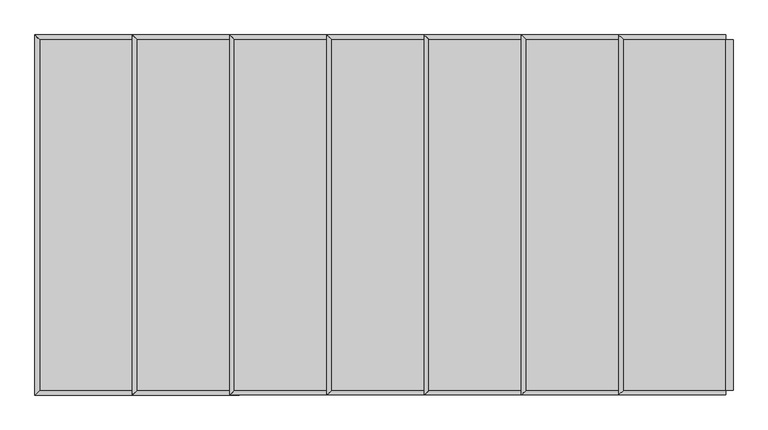
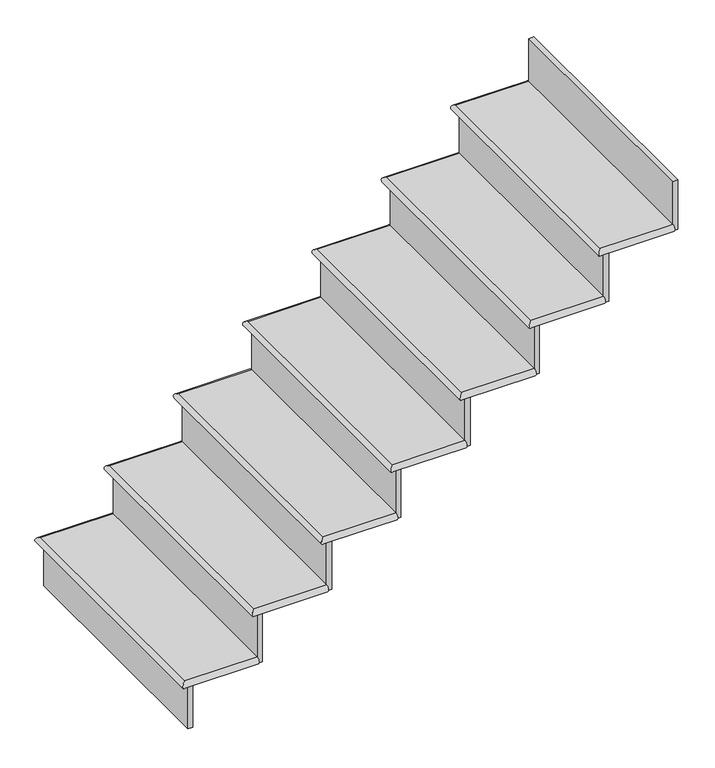
"""IFC4 building model written with IfcOpenShell, lengths in millimetres: stair flight geometry."""

import ifcopenshell
import ifcopenshell.guid

model = None  # the IFC model being written
_history = None  # IfcOwnerHistory: only IFC2X3 demands one
_inside = {}  # id of a spatial element -> (the spatial element, [elements in it])
_under = {}  # id of a project, library or spatial element -> (it, [spatial elements below it])
_declared = {}  # id of a project -> (the project, [libraries it declares])
_typed = {}  # id of a type object -> (the type object, [elements of that type])
_made_of = {}  # id of a material, layer set ... -> (it, [elements and type objects made of it])


def new_model(schema):
    """Start an empty IFC model of exactly this schema.

    Asked for "IFC4X3", IfcOpenShell would pick the latest addendum, in which some entities
    have other attributes; the version numbers below select the first issue.
    IFC2X3 requires an IfcOwnerHistory on every rooted entity: one is made here for all.
    """
    global model, _history
    if schema == "IFC4X3":
        model = ifcopenshell.file(schema_version=(4, 3, 0, 0))
    else:
        model = ifcopenshell.file(schema=schema)
    _inside.clear()
    _under.clear()
    _declared.clear()
    _typed.clear()
    _made_of.clear()
    _history = None
    if model.schema == "IFC2X3":
        org = make("IfcOrganization", Name="unknown")
        user = make(
            "IfcPersonAndOrganization",
            ThePerson=make("IfcPerson", FamilyName="unknown"),
            TheOrganization=org,
        )
        app = make(
            "IfcApplication",
            ApplicationDeveloper=org,
            Version="unknown",
            ApplicationFullName="unknown",
            ApplicationIdentifier="unknown",
        )
        _history = make(
            "IfcOwnerHistory",
            OwningUser=user,
            OwningApplication=app,
            ChangeAction="ADDED",
            CreationDate=0,
        )
    return model


def make(cls, **values):
    """One entity of the class cls with the attributes given. An attribute that is None is left unset."""
    return model.create_entity(
        cls, **{name: value for name, value in values.items() if value is not None}
    )


def rooted(cls, **values):
    """An entity with a GlobalId (a new one), such as an element, a storey or a relation."""
    return make(cls, GlobalId=ifcopenshell.guid.new(), OwnerHistory=_history, **values)


def si_unit(unit_type, name, prefix=None):
    """IfcSIUnit, for example si_unit("LENGTHUNIT", "METRE", prefix="MILLI")."""
    return make("IfcSIUnit", UnitType=unit_type, Prefix=prefix, Name=name)


def assignment(units):
    """IfcUnitAssignment: the units of a project."""
    return None if units is None else make("IfcUnitAssignment", Units=units)


def point(xyz):
    """IfcCartesianPoint."""
    return None if xyz is None else make("IfcCartesianPoint", Coordinates=xyz)


def direction(xyz):
    """IfcDirection."""
    return None if xyz is None else make("IfcDirection", DirectionRatios=xyz)


def frame(location, z_axis=None, x_axis=None):
    """IfcAxis2Placement3D, a coordinate frame: its origin and axes. An axis left out is left unset."""
    return make(
        "IfcAxis2Placement3D",
        Location=point(location),
        Axis=direction(z_axis),
        RefDirection=direction(x_axis),
    )


def origin():
    """The frame at (0, 0, 0) with its axes left unset."""
    return frame((0.0, 0.0, 0.0))


def place(relative_to, where):
    """IfcLocalPlacement: puts the frame where relative to a parent placement (None: the world)."""
    return make(
        "IfcLocalPlacement", PlacementRelTo=relative_to, RelativePlacement=where
    )


def context(
    kind, dimensions, precision=None, world=None, true_north=None, identifier=None
):
    """IfcGeometricRepresentationContext, for example the 3D "Model" context."""
    return make(
        "IfcGeometricRepresentationContext",
        ContextIdentifier=identifier,
        ContextType=kind,
        CoordinateSpaceDimension=dimensions,
        Precision=precision,
        WorldCoordinateSystem=world,
        TrueNorth=true_north,
    )


def project(units=None, contexts=None):
    """IfcProject with its units and contexts."""
    return rooted(
        "IfcProject",
        Name="project",
        RepresentationContexts=contexts,
        UnitsInContext=assignment(units),
    )


def spatial(cls, under=None, at=None, **own):
    """A site, building, storey or space (cls), placed at a placement, below another one or the project."""
    s = rooted(cls, ObjectPlacement=at, **own)
    if under is not None:
        _under.setdefault(under.id(), (under, []))[1].append(s)
    return s


def circle_curve(where, radius):
    """IfcCircle in the frame where."""
    return make("IfcCircle", Position=where, Radius=radius)


def ellipse_curve(where, semi_axis1, semi_axis2):
    """IfcEllipse in the frame where."""
    return make(
        "IfcEllipse", Position=where, SemiAxis1=semi_axis1, SemiAxis2=semi_axis2
    )


def faces_of(points, faces, orient=None, outer=None):
    """IfcFace entities. A face is a list of loops; a loop is a list of indices into points, from 0.

    orient and outer hold one flag for each loop. By default every Orientation is true, the
    first loop of a face is its IfcFaceOuterBound and the others are IfcFaceBound.
    """
    made = []
    for i, loops in enumerate(faces):
        bounds = []
        for j, loop in enumerate(loops):
            is_outer = j == 0 if outer is None else outer[i][j]
            bounds.append(
                make(
                    "IfcFaceOuterBound" if is_outer else "IfcFaceBound",
                    Bound=make("IfcPolyLoop", Polygon=[points[k] for k in loop]),
                    Orientation=True if orient is None else orient[i][j],
                )
            )
        made.append(make("IfcFace", Bounds=bounds))
    return made


def faceted_brep(points, faces, orient=None, outer=None, voids=None):
    """IfcFacetedBrep: a solid bounded by flat faces; with voids (closed shells), ...WithVoids."""
    shared = [point(p) for p in points]
    hull = make("IfcClosedShell", CfsFaces=faces_of(shared, faces, orient, outer))
    if voids is None:
        return make("IfcFacetedBrep", Outer=hull)
    return make(
        "IfcFacetedBrepWithVoids",
        Outer=hull,
        Voids=[
            make(cls, CfsFaces=faces_of(shared, fs, o, b)) for cls, fs, o, b in voids
        ],
    )


def shape(context_of_items, identifier, shape_type, items):
    """IfcShapeRepresentation: the items that make up one representation, for example the "Body"."""
    return make(
        "IfcShapeRepresentation",
        ContextOfItems=context_of_items,
        RepresentationIdentifier=identifier,
        RepresentationType=shape_type,
        Items=items,
    )


def source(mapping_origin, context_of_items, identifier, shape_type, items):
    """IfcRepresentationMap: a shape defined once, which mapped items show again and again."""
    return make(
        "IfcRepresentationMap",
        MappingOrigin=mapping_origin,
        MappedRepresentation=shape(context_of_items, identifier, shape_type, items),
    )


def transform(
    local_origin,
    x_axis=None,
    y_axis=None,
    z_axis=None,
    scale=None,
    scale2=None,
    scale3=None,
    uniform=True,
):
    """IfcCartesianTransformationOperator3D, or its non-uniform kind. x_axis, y_axis, z_axis: its Axis1, 2, 3."""
    if uniform:
        return make(
            "IfcCartesianTransformationOperator3D",
            Axis1=direction(x_axis),
            Axis2=direction(y_axis),
            LocalOrigin=point(local_origin),
            Scale=scale,
            Axis3=direction(z_axis),
        )
    return make(
        "IfcCartesianTransformationOperator3DnonUniform",
        Axis1=direction(x_axis),
        Axis2=direction(y_axis),
        LocalOrigin=point(local_origin),
        Scale=scale,
        Axis3=direction(z_axis),
        Scale2=scale2,
        Scale3=scale3,
    )


def mapped(mapping_source, mapping_target):
    """IfcMappedItem: shows the shape of a source again, moved by a transform."""
    return make(
        "IfcMappedItem", MappingSource=mapping_source, MappingTarget=mapping_target
    )


def made_of(thing, what):
    """Note that an element or type object is made of a material, layer set ...; save() writes the relation."""
    if what is not None:
        _made_of.setdefault(what.id(), (what, []))[1].append(thing)
    return thing


def element(
    cls,
    number,
    at=None,
    inside=None,
    cuts=None,
    type_object=None,
    material=None,
    context=None,
    identifier="Body",
    shape_type=None,
    held_by="IfcProductDefinitionShape",
    body=None,
    shapes=None,
    **own,
):
    """One element of the class cls, such as IfcWall. Its Tag is "e" and its number.

    at: its placement. inside: the storey or other place that contains it. cuts: it is an
    opening in that element (IfcRelVoidsElement). A single representation is given by context,
    identifier, shape_type and body (its items); several are given by shapes. held_by: the class
    of the entity that holds the representations. save() writes the other relations.
    """
    e = rooted(cls, Tag="e%d" % number, ObjectPlacement=at, **own)
    if body is not None:
        shapes = [shape(context, identifier, shape_type, body)]
    if shapes is not None:
        e.Representation = make(held_by, Representations=shapes)
    if inside is not None:
        _inside.setdefault(inside.id(), (inside, []))[1].append(e)
    if cuts is not None:
        rooted(
            "IfcRelVoidsElement", RelatingBuildingElement=cuts, RelatedOpeningElement=e
        )
    if type_object is not None:
        _typed.setdefault(type_object.id(), (type_object, []))[1].append(e)
    return made_of(e, material)


def aggregate(whole, parts):
    """IfcRelAggregates: a whole, such as a stair, and the parts it consists of."""
    return rooted("IfcRelAggregates", RelatingObject=whole, RelatedObjects=parts)


def save(model, path):
    """Write the relations noted so far, then the file.

    IfcRelAggregates (storeys below a building ...), IfcRelContainedInSpatialStructure (elements
    in a storey), IfcRelDefinesByType, IfcRelAssociatesMaterial and IfcRelDeclares: one each for
    every whole, place, type object, material and project.
    """
    for whole, parts in _under.values():
        aggregate(whole, parts)
    for where, things in _inside.values():
        rooted(
            "IfcRelContainedInSpatialStructure",
            RelatedElements=things,
            RelatingStructure=where,
        )
    for kind, things in _typed.values():
        rooted("IfcRelDefinesByType", RelatedObjects=things, RelatingType=kind)
    for what, things in _made_of.values():
        rooted("IfcRelAssociatesMaterial", RelatedObjects=things, RelatingMaterial=what)
    for by, libraries in _declared.values():
        rooted("IfcRelDeclares", RelatingContext=by, RelatedDefinitions=libraries)
    model.write(path)


def plane_surface(at):
    """IfcPlane: the flat surface through the origin of the frame at, square to its z axis."""
    return make("IfcPlane", Position=at)


def cylinder_surface(at, radius):
    """IfcCylindricalSurface: all points at the distance radius from the z axis of the frame at."""
    return make("IfcCylindricalSurface", Position=at, Radius=radius)


def advanced_brep(points, edges, surfaces, faces):
    """IfcAdvancedBrep: a solid bounded by faces that lie on surfaces and meet in shared edges.

    An edge is (start, end): straight between two places in points (the first is 0);
    or (start, end, curve); or (start, end, curve, False) where it runs against its curve.
    A face is (place in surfaces, loops), or (place, loops, False) where it looks against
    its surface's normal. A loop lists edges by number (the first is 1), with a minus sign
    where the edge is run from its end to its start. The first loop is the outer one.
    """
    corners = [point(p) for p in points]
    vertices = [make("IfcVertexPoint", VertexGeometry=c) for c in corners]
    made = []
    for start, end, *more in edges:
        made.append(
            make(
                "IfcEdgeCurve",
                EdgeStart=vertices[start],
                EdgeEnd=vertices[end],
                EdgeGeometry=more[0] if more else make("IfcPolyline", Points=[corners[start], corners[end]]),
                SameSense=more[1] if len(more) > 1 else True,
            )
        )
    hull = []
    for where, loops, *sense in faces:
        bounds = []
        for j, loop in enumerate(loops):
            ring = [make("IfcOrientedEdge", EdgeElement=made[abs(k) - 1], Orientation=k > 0) for k in loop]
            bounds.append(
                make(
                    "IfcFaceOuterBound" if j == 0 else "IfcFaceBound",
                    Bound=make("IfcEdgeLoop", EdgeList=ring),
                    Orientation=True,
                )
            )
        hull.append(make("IfcAdvancedFace", Bounds=bounds, FaceSurface=surfaces[where], SameSense=sense[0] if sense else True))
    return make("IfcAdvancedBrep", Outer=make("IfcClosedShell", CfsFaces=hull))


def stair_flight_e1e404fc(model_context):
    return source(origin(), model_context, "Body", "SolidModel", [
        advanced_brep(
        [(-17769.3481446, 3955.9128094, 165.1), (-17769.3481446, 3955.9128094, 190.5), (-17769.3481446, 4870.3128094, 190.5), (-17769.3481446, 4870.3128094, 165.1), (-17502.6481446, 3955.9128094, 190.5), (-17502.6481446, 4870.3128094, 190.5), (-17502.6481446, 4870.3128094, 165.1), (-17502.6481446, 3955.9128094, 165.1)],
        [
            (0, 1, ellipse_curve(frame((-17769.3481446, 3955.9128094, 177.8), z_axis=(-0.7071067811865449, 0.7071067811865502, 0.0), x_axis=(-0.7071067811865503, -0.7071067811865447, 0.0)), 17.9605122, 12.7)),
            (1, 2),
            (2, 3, ellipse_curve(frame((-17769.3481446, 4870.3128094, 177.8), z_axis=(-0.7071067811865501, -0.7071067811865447, 0.0), x_axis=(0.7071067811865446, -0.7071067811865506, 0.0)), 17.9605122, 12.7)),
            (3, 0),
            (4, 5),
            (5, 2),
            (1, 4),
            (6, 7),
            (7, 0),
            (3, 6),
            (4, 7, circle_curve(frame((-17502.6481446, 3955.9128094, 177.8), z_axis=(1.0, 0.0, 0.0), x_axis=(0.0, 1.0, 0.0)), 12.7)),
            (6, 5, circle_curve(frame((-17502.6481446, 4870.3128094, 177.8), z_axis=(1.0, 0.0, 0.0), x_axis=(0.0, -1.0, 0.0)), 12.7)),
        ],
        [
            cylinder_surface(frame((-17769.3481446, 3955.9128094, 177.8), z_axis=(0.0, -1.0, 0.0), x_axis=(1.0, 0.0, 0.0)), 12.7),
            plane_surface(frame((-17782.0481446, 4870.3128094, 190.5), z_axis=(0.0, 0.0, 1.0), x_axis=(-1.0, 0.0, 0.0))),
            plane_surface(frame((-17782.0481446, 4870.3128094, 165.1), z_axis=(0.0, 0.0, -1.0), x_axis=(1.0, 0.0, 0.0))),
            plane_surface(frame((-17502.6481446, 3955.9128094, 190.5), z_axis=(1.0, 0.0, 0.0), x_axis=(0.0, 0.0, -1.0))),
            cylinder_surface(frame((-17502.6481446, 3955.9128094, 177.8), z_axis=(1.0, 0.0, 0.0), x_axis=(0.0, 1.0, 0.0)), 12.7),
            cylinder_surface(frame((-17769.3481446, 4870.3128094, 177.8), z_axis=(-1.0, 0.0, 0.0), x_axis=(0.0, -1.0, 0.0)), 12.7),
        ],
        [
            (0, [[1, 2, 3, 4]]),
            (1, [[5, 6, -2, 7]]),
            (2, [[8, 9, -4, 10]]),
            (3, [[-5, 11, -8, 12]]),
            (4, [[-11, -7, -1, -9]]),
            (5, [[-3, -6, -12, -10]]),
        ],
    ),
        faceted_brep([(-17756.6481446, 3955.9128094, 165.1), (-17756.6481446, 3955.9128094, 0.0), (-17737.5981446, 3955.9128094, 0.0), (-17737.5981446, 3955.9128094, 165.1), (-17756.6481446, 4870.3128094, 165.1), (-17737.5981446, 4870.3128094, 165.1), (-17737.5981446, 4870.3128094, 0.0), (-17756.6481446, 4870.3128094, 0.0)], [[[0, 1, 2, 3]], [[4, 5, 6, 7]], [[1, 0, 4, 7]], [[2, 1, 7, 6]], [[3, 2, 6, 5]], [[0, 3, 5, 4]]]),
        faceted_brep([(-17502.6481446, 3955.9128094, 355.6), (-17502.6481446, 3955.9128094, 165.1), (-17483.5981446, 3955.9128094, 165.1), (-17483.5981446, 3955.9128094, 355.6), (-17502.6481446, 4870.3128094, 355.6), (-17483.5981446, 4870.3128094, 355.6), (-17483.5981446, 4870.3128094, 165.1), (-17502.6481446, 4870.3128094, 165.1)], [[[0, 1, 2, 3]], [[4, 5, 6, 7]], [[1, 0, 4, 7]], [[2, 1, 7, 6]], [[3, 2, 6, 5]], [[0, 3, 5, 4]]]),
        advanced_brep(
        [(-17248.6481446, 3955.9128094, 381.0), (-17248.6481446, 4870.3128094, 381.0), (-17515.3481446, 4870.3128094, 381.0), (-17515.3481446, 3955.9128094, 381.0), (-17248.6481446, 4870.3128094, 355.6), (-17248.6481446, 3955.9128094, 355.6), (-17515.3481446, 3955.9128094, 355.6), (-17515.3481446, 4870.3128094, 355.6)],
        [
            (0, 1),
            (1, 2),
            (2, 3),
            (3, 0),
            (4, 5),
            (5, 6),
            (6, 7),
            (7, 4),
            (0, 5, circle_curve(frame((-17248.6481446, 3955.9128094, 368.3), z_axis=(1.0, 0.0, 0.0), x_axis=(0.0, 1.0, 0.0)), 12.7)),
            (4, 1, circle_curve(frame((-17248.6481446, 4870.3128094, 368.3), z_axis=(1.0, 0.0, 0.0), x_axis=(0.0, -1.0, 0.0)), 12.7)),
            (6, 3, ellipse_curve(frame((-17515.3481446, 3955.9128094, 368.3), z_axis=(-0.7071067811865457, 0.7071067811865495, 0.0), x_axis=(-0.7071067811865496, -0.7071067811865455, 0.0)), 17.9605122, 12.7)),
            (2, 7, ellipse_curve(frame((-17515.3481446, 4870.3128094, 368.3), z_axis=(-0.7071067811865496, -0.7071067811865455, 0.0), x_axis=(0.7071067811865455, -0.7071067811865496, 0.0)), 17.9605122, 12.7)),
        ],
        [
            plane_surface(frame((-17782.0481446, 4870.3128094, 381.0), z_axis=(0.0, 0.0, 1.0), x_axis=(-1.0, 0.0, 0.0))),
            plane_surface(frame((-17782.0481446, 4870.3128094, 355.6), z_axis=(0.0, 0.0, -1.0), x_axis=(1.0, 0.0, 0.0))),
            plane_surface(frame((-17248.6481446, 3955.9128094, 381.0), z_axis=(1.0, 0.0, 0.0), x_axis=(0.0, 0.0, -1.0))),
            cylinder_surface(frame((-17515.3481446, 3955.9128094, 368.3), z_axis=(0.0, -1.0, 0.0), x_axis=(1.0, 0.0, 0.0)), 12.7),
            cylinder_surface(frame((-17248.6481446, 3955.9128094, 368.3), z_axis=(1.0, 0.0, 0.0), x_axis=(0.0, 1.0, 0.0)), 12.7),
            cylinder_surface(frame((-17515.3481446, 4870.3128094, 368.3), z_axis=(-1.0, 0.0, 0.0), x_axis=(0.0, -1.0, 0.0)), 12.7),
        ],
        [
            (0, [[1, 2, 3, 4]]),
            (1, [[5, 6, 7, 8]]),
            (2, [[-1, 9, -5, 10]]),
            (3, [[11, -3, 12, -7]]),
            (4, [[-9, -4, -11, -6]]),
            (5, [[-12, -2, -10, -8]]),
        ],
    ),
        faceted_brep([(-17248.6481446, 3955.9128094, 546.1), (-17248.6481446, 3955.9128094, 355.6), (-17229.5981446, 3955.9128094, 355.6), (-17229.5981446, 3955.9128094, 546.1), (-17248.6481446, 4870.3128094, 546.1), (-17229.5981446, 4870.3128094, 546.1), (-17229.5981446, 4870.3128094, 355.6), (-17248.6481446, 4870.3128094, 355.6)], [[[0, 1, 2, 3]], [[4, 5, 6, 7]], [[1, 0, 4, 7]], [[2, 1, 7, 6]], [[3, 2, 6, 5]], [[0, 3, 5, 4]]]),
        advanced_brep(
        [(-16994.6481446, 3955.9128094, 571.5), (-16994.6481446, 4870.3128094, 571.5), (-17261.3481446, 4870.3128094, 571.5), (-17261.3481446, 3955.9128094, 571.5), (-16994.6481446, 4870.3128094, 546.1), (-16994.6481446, 3955.9128094, 546.1), (-17261.3481446, 3955.9128094, 546.1), (-17261.3481446, 4870.3128094, 546.1)],
        [
            (0, 1),
            (1, 2),
            (2, 3),
            (3, 0),
            (4, 5),
            (5, 6),
            (6, 7),
            (7, 4),
            (0, 5, circle_curve(frame((-16994.6481446, 3955.9128094, 558.8), z_axis=(1.0, 0.0, 0.0), x_axis=(0.0, 1.0, 0.0)), 12.7)),
            (4, 1, circle_curve(frame((-16994.6481446, 4870.3128094, 558.8), z_axis=(1.0, 0.0, 0.0), x_axis=(0.0, -1.0, 0.0)), 12.7)),
            (6, 3, ellipse_curve(frame((-17261.3481446, 3955.9128094, 558.8), z_axis=(-0.7071067811865457, 0.7071067811865495, 0.0), x_axis=(-0.7071067811865496, -0.7071067811865455, 0.0)), 17.9605122, 12.7)),
            (2, 7, ellipse_curve(frame((-17261.3481446, 4870.3128094, 558.8), z_axis=(-0.7071067811865496, -0.7071067811865455, 0.0), x_axis=(0.7071067811865455, -0.7071067811865496, 0.0)), 17.9605122, 12.7)),
        ],
        [
            plane_surface(frame((-17528.0481446, 4870.3128094, 571.5), z_axis=(0.0, 0.0, 1.0), x_axis=(-1.0, 0.0, 0.0))),
            plane_surface(frame((-17528.0481446, 4870.3128094, 546.1), z_axis=(0.0, 0.0, -1.0), x_axis=(1.0, 0.0, 0.0))),
            plane_surface(frame((-16994.6481446, 3955.9128094, 571.5), z_axis=(1.0, 0.0, 0.0), x_axis=(0.0, 0.0, -1.0))),
            cylinder_surface(frame((-17261.3481446, 3955.9128094, 558.8), z_axis=(0.0, -1.0, 0.0), x_axis=(1.0, 0.0, 0.0)), 12.7),
            cylinder_surface(frame((-16994.6481446, 3955.9128094, 558.8), z_axis=(1.0, 0.0, 0.0), x_axis=(0.0, 1.0, 0.0)), 12.7),
            cylinder_surface(frame((-17261.3481446, 4870.3128094, 558.8), z_axis=(-1.0, 0.0, 0.0), x_axis=(0.0, -1.0, 0.0)), 12.7),
        ],
        [
            (0, [[1, 2, 3, 4]]),
            (1, [[5, 6, 7, 8]]),
            (2, [[-1, 9, -5, 10]]),
            (3, [[11, -3, 12, -7]]),
            (4, [[-9, -4, -11, -6]]),
            (5, [[-12, -2, -10, -8]]),
        ],
    ),
        faceted_brep([(-16994.6481446, 3955.9128094, 736.6), (-16994.6481446, 3955.9128094, 546.1), (-16975.5981446, 3955.9128094, 546.1), (-16975.5981446, 3955.9128094, 736.6), (-16994.6481446, 4870.3128094, 736.6), (-16975.5981446, 4870.3128094, 736.6), (-16975.5981446, 4870.3128094, 546.1), (-16994.6481446, 4870.3128094, 546.1)], [[[0, 1, 2, 3]], [[4, 5, 6, 7]], [[1, 0, 4, 7]], [[2, 1, 7, 6]], [[3, 2, 6, 5]], [[0, 3, 5, 4]]]),
        advanced_brep(
        [(-16740.6481446, 3955.9128094, 762.0), (-16740.6481446, 4870.3128094, 762.0), (-17007.3481446, 4870.3128094, 762.0), (-17007.3481446, 3955.9128094, 762.0), (-16740.6481446, 4870.3128094, 736.6), (-16740.6481446, 3955.9128094, 736.6), (-17007.3481446, 3955.9128094, 736.6), (-17007.3481446, 4870.3128094, 736.6)],
        [
            (0, 1),
            (1, 2),
            (2, 3),
            (3, 0),
            (4, 5),
            (5, 6),
            (6, 7),
            (7, 4),
            (0, 5, circle_curve(frame((-16740.6481446, 3955.9128094, 749.3), z_axis=(1.0, 0.0, 0.0), x_axis=(0.0, 1.0, 0.0)), 12.7)),
            (4, 1, circle_curve(frame((-16740.6481446, 4870.3128094, 749.3), z_axis=(1.0, 0.0, 0.0), x_axis=(0.0, -1.0, 0.0)), 12.7)),
            (6, 3, ellipse_curve(frame((-17007.3481446, 3955.9128094, 749.3), z_axis=(-0.7071067811865457, 0.7071067811865495, 0.0), x_axis=(-0.7071067811865496, -0.7071067811865455, 0.0)), 17.9605122, 12.7)),
            (2, 7, ellipse_curve(frame((-17007.3481446, 4870.3128094, 749.3), z_axis=(-0.7071067811865496, -0.7071067811865455, 0.0), x_axis=(0.7071067811865455, -0.7071067811865496, 0.0)), 17.9605122, 12.7)),
        ],
        [
            plane_surface(frame((-17274.0481446, 4870.3128094, 762.0), z_axis=(0.0, 0.0, 1.0), x_axis=(-1.0, 0.0, 0.0))),
            plane_surface(frame((-17274.0481446, 4870.3128094, 736.6), z_axis=(0.0, 0.0, -1.0), x_axis=(1.0, 0.0, 0.0))),
            plane_surface(frame((-16740.6481446, 3955.9128094, 762.0), z_axis=(1.0, 0.0, 0.0), x_axis=(0.0, 0.0, -1.0))),
            cylinder_surface(frame((-17007.3481446, 3955.9128094, 749.3), z_axis=(0.0, -1.0, 0.0), x_axis=(1.0, 0.0, 0.0)), 12.7),
            cylinder_surface(frame((-16740.6481446, 3955.9128094, 749.3), z_axis=(1.0, 0.0, 0.0), x_axis=(0.0, 1.0, 0.0)), 12.7),
            cylinder_surface(frame((-17007.3481446, 4870.3128094, 749.3), z_axis=(-1.0, 0.0, 0.0), x_axis=(0.0, -1.0, 0.0)), 12.7),
        ],
        [
            (0, [[1, 2, 3, 4]]),
            (1, [[5, 6, 7, 8]]),
            (2, [[-1, 9, -5, 10]]),
            (3, [[11, -3, 12, -7]]),
            (4, [[-9, -4, -11, -6]]),
            (5, [[-12, -2, -10, -8]]),
        ],
    ),
        faceted_brep([(-16740.6481446, 3955.9128094, 927.1), (-16740.6481446, 3955.9128094, 736.6), (-16721.5981446, 3955.9128094, 736.6), (-16721.5981446, 3955.9128094, 927.1), (-16740.6481446, 4870.3128094, 927.1), (-16721.5981446, 4870.3128094, 927.1), (-16721.5981446, 4870.3128094, 736.6), (-16740.6481446, 4870.3128094, 736.6)], [[[0, 1, 2, 3]], [[4, 5, 6, 7]], [[1, 0, 4, 7]], [[2, 1, 7, 6]], [[3, 2, 6, 5]], [[0, 3, 5, 4]]]),
        advanced_brep(
        [(-16486.6481446, 3955.9128094, 952.5), (-16486.6481446, 4870.3128094, 952.5), (-16753.3481446, 4870.3128094, 952.5), (-16753.3481446, 3955.9128094, 952.5), (-16486.6481446, 4870.3128094, 927.1), (-16486.6481446, 3955.9128094, 927.1), (-16753.3481446, 3955.9128094, 927.1), (-16753.3481446, 4870.3128094, 927.1)],
        [
            (0, 1),
            (1, 2),
            (2, 3),
            (3, 0),
            (4, 5),
            (5, 6),
            (6, 7),
            (7, 4),
            (0, 5, circle_curve(frame((-16486.6481446, 3955.9128094, 939.8), z_axis=(1.0, 0.0, 0.0), x_axis=(0.0, 1.0, 0.0)), 12.7)),
            (4, 1, circle_curve(frame((-16486.6481446, 4870.3128094, 939.8), z_axis=(1.0, 0.0, 0.0), x_axis=(0.0, -1.0, 0.0)), 12.7)),
            (6, 3, ellipse_curve(frame((-16753.3481446, 3955.9128094, 939.8), z_axis=(-0.7071067811865457, 0.7071067811865495, 0.0), x_axis=(-0.7071067811865496, -0.7071067811865455, 0.0)), 17.9605122, 12.7)),
            (2, 7, ellipse_curve(frame((-16753.3481446, 4870.3128094, 939.8), z_axis=(-0.7071067811865496, -0.7071067811865455, 0.0), x_axis=(0.7071067811865455, -0.7071067811865496, 0.0)), 17.9605122, 12.7)),
        ],
        [
            plane_surface(frame((-17020.0481446, 4870.3128094, 952.5), z_axis=(0.0, 0.0, 1.0), x_axis=(-1.0, 0.0, 0.0))),
            plane_surface(frame((-17020.0481446, 4870.3128094, 927.1), z_axis=(0.0, 0.0, -1.0), x_axis=(1.0, 0.0, 0.0))),
            plane_surface(frame((-16486.6481446, 3955.9128094, 952.5), z_axis=(1.0, 0.0, 0.0), x_axis=(0.0, 0.0, -1.0))),
            cylinder_surface(frame((-16753.3481446, 3955.9128094, 939.8), z_axis=(0.0, -1.0, 0.0), x_axis=(1.0, 0.0, 0.0)), 12.7),
            cylinder_surface(frame((-16486.6481446, 3955.9128094, 939.8), z_axis=(1.0, 0.0, 0.0), x_axis=(0.0, 1.0, 0.0)), 12.7),
            cylinder_surface(frame((-16753.3481446, 4870.3128094, 939.8), z_axis=(-1.0, 0.0, 0.0), x_axis=(0.0, -1.0, 0.0)), 12.7),
        ],
        [
            (0, [[1, 2, 3, 4]]),
            (1, [[5, 6, 7, 8]]),
            (2, [[-1, 9, -5, 10]]),
            (3, [[11, -3, 12, -7]]),
            (4, [[-9, -4, -11, -6]]),
            (5, [[-12, -2, -10, -8]]),
        ],
    ),
        faceted_brep([(-16486.6481446, 3955.9128094, 1117.6), (-16486.6481446, 3955.9128094, 927.1), (-16467.5981446, 3955.9128094, 927.1), (-16467.5981446, 3955.9128094, 1117.6), (-16486.6481446, 4870.3128094, 1117.6), (-16467.5981446, 4870.3128094, 1117.6), (-16467.5981446, 4870.3128094, 927.1), (-16486.6481446, 4870.3128094, 927.1)], [[[0, 1, 2, 3]], [[4, 5, 6, 7]], [[1, 0, 4, 7]], [[2, 1, 7, 6]], [[3, 2, 6, 5]], [[0, 3, 5, 4]]]),
        advanced_brep(
        [(-16232.6481446, 3955.9128094, 1143.0), (-16232.6481446, 4870.3128094, 1143.0), (-16499.3481446, 4870.3128094, 1143.0), (-16499.3481446, 3955.9128094, 1143.0), (-16232.6481446, 4870.3128094, 1117.6), (-16232.6481446, 3955.9128094, 1117.6), (-16499.3481446, 3955.9128094, 1117.6), (-16499.3481446, 4870.3128094, 1117.6)],
        [
            (0, 1),
            (1, 2),
            (2, 3),
            (3, 0),
            (4, 5),
            (5, 6),
            (6, 7),
            (7, 4),
            (0, 5, circle_curve(frame((-16232.6481446, 3955.9128094, 1130.3), z_axis=(1.0, 0.0, 0.0), x_axis=(0.0, 1.0, 0.0)), 12.7)),
            (4, 1, circle_curve(frame((-16232.6481446, 4870.3128094, 1130.3), z_axis=(1.0, 0.0, 0.0), x_axis=(0.0, -1.0, 0.0)), 12.7)),
            (6, 3, ellipse_curve(frame((-16499.3481446, 3955.9128094, 1130.3), z_axis=(-0.7071067811865457, 0.7071067811865495, 0.0), x_axis=(-0.7071067811865496, -0.7071067811865455, 0.0)), 17.9605122, 12.7)),
            (2, 7, ellipse_curve(frame((-16499.3481446, 4870.3128094, 1130.3), z_axis=(-0.7071067811865496, -0.7071067811865455, 0.0), x_axis=(0.7071067811865455, -0.7071067811865496, 0.0)), 17.9605122, 12.7)),
        ],
        [
            plane_surface(frame((-16766.0481446, 4870.3128094, 1143.0), z_axis=(0.0, 0.0, 1.0), x_axis=(-1.0, 0.0, 0.0))),
            plane_surface(frame((-16766.0481446, 4870.3128094, 1117.6), z_axis=(0.0, 0.0, -1.0), x_axis=(1.0, 0.0, 0.0))),
            plane_surface(frame((-16232.6481446, 3955.9128094, 1143.0), z_axis=(1.0, 0.0, 0.0), x_axis=(0.0, 0.0, -1.0))),
            cylinder_surface(frame((-16499.3481446, 3955.9128094, 1130.3), z_axis=(0.0, -1.0, 0.0), x_axis=(1.0, 0.0, 0.0)), 12.7),
            cylinder_surface(frame((-16232.6481446, 3955.9128094, 1130.3), z_axis=(1.0, 0.0, 0.0), x_axis=(0.0, 1.0, 0.0)), 12.7),
            cylinder_surface(frame((-16499.3481446, 4870.3128094, 1130.3), z_axis=(-1.0, 0.0, 0.0), x_axis=(0.0, -1.0, 0.0)), 12.7),
        ],
        [
            (0, [[1, 2, 3, 4]]),
            (1, [[5, 6, 7, 8]]),
            (2, [[-1, 9, -5, 10]]),
            (3, [[11, -3, 12, -7]]),
            (4, [[-9, -4, -11, -6]]),
            (5, [[-12, -2, -10, -8]]),
        ],
    ),
        faceted_brep([(-15978.6481446, 3955.9128094, 1498.6), (-15978.6481446, 3955.9128094, 1308.1), (-15959.5981446, 3955.9128094, 1308.1), (-15959.5981446, 3955.9128094, 1498.6), (-15978.6481446, 4870.3128094, 1498.6), (-15959.5981446, 4870.3128094, 1498.6), (-15959.5981446, 4870.3128094, 1308.1), (-15978.6481446, 4870.3128094, 1308.1)], [[[0, 1, 2, 3]], [[4, 5, 6, 7]], [[1, 0, 4, 7]], [[2, 1, 7, 6]], [[3, 2, 6, 5]], [[0, 3, 5, 4]]]),
        faceted_brep([(-16232.6481446, 3955.9128094, 1308.1), (-16232.6481446, 3955.9128094, 1117.6), (-16213.5981446, 3955.9128094, 1117.6), (-16213.5981446, 3955.9128094, 1308.1), (-16232.6481446, 4870.3128094, 1308.1), (-16213.5981446, 4870.3128094, 1308.1), (-16213.5981446, 4870.3128094, 1117.6), (-16232.6481446, 4870.3128094, 1117.6)], [[[0, 1, 2, 3]], [[4, 5, 6, 7]], [[1, 0, 4, 7]], [[2, 1, 7, 6]], [[3, 2, 6, 5]], [[0, 3, 5, 4]]]),
        advanced_brep(
        [(-15978.6481446, 3955.9128094, 1333.5), (-15978.6481446, 4870.3128094, 1333.5), (-16245.3481446, 4870.3128094, 1333.5), (-16245.3481446, 3955.9128094, 1333.5), (-16004.0481446, 3955.9128094, 1333.5), (-15978.6481446, 4870.3128094, 1308.1), (-15978.6481446, 3955.9128094, 1308.1), (-16004.0481446, 3955.9128094, 1308.1), (-16245.3481446, 3955.9128094, 1308.1), (-16245.3481446, 4870.3128094, 1308.1)],
        [
            (0, 1),
            (1, 2),
            (2, 3),
            (3, 4),
            (4, 0),
            (5, 6),
            (6, 7),
            (7, 8),
            (8, 9),
            (9, 5),
            (0, 6, circle_curve(frame((-15978.6481446, 3955.9128094, 1320.8), z_axis=(1.0, 0.0, 0.0), x_axis=(0.0, 1.0, 0.0)), 12.7)),
            (5, 1, circle_curve(frame((-15978.6481446, 4870.3128094, 1320.8), z_axis=(1.0, 0.0, 0.0), x_axis=(0.0, -1.0, 0.0)), 12.7)),
            (8, 3, ellipse_curve(frame((-16245.3481446, 3955.9128094, 1320.8), z_axis=(-0.7071067811865455, 0.7071067811865496, 0.0), x_axis=(-0.7071067811865496, -0.7071067811865455, 0.0)), 17.9605122, 12.7)),
            (2, 9, ellipse_curve(frame((-16245.3481446, 4870.3128094, 1320.8), z_axis=(-0.7071067811865496, -0.7071067811865455, 0.0), x_axis=(0.7071067811865455, -0.7071067811865496, 0.0)), 17.9605122, 12.7)),
        ],
        [
            plane_surface(frame((-17782.0481446, 4870.3128094, 1333.5), z_axis=(0.0, 0.0, 1.0), x_axis=(-1.0, 0.0, 0.0))),
            plane_surface(frame((-17782.0481446, 4870.3128094, 1308.1), z_axis=(0.0, 0.0, -1.0), x_axis=(1.0, 0.0, 0.0))),
            plane_surface(frame((-15978.6481446, 3955.9128094, 1333.5), z_axis=(1.0, 0.0, 0.0), x_axis=(0.0, 0.0, -1.0))),
            cylinder_surface(frame((-16245.3481446, 3955.9128094, 1320.8), z_axis=(0.0, -1.0, 0.0), x_axis=(1.0, 0.0, 0.0)), 12.7),
            cylinder_surface(frame((-15978.6481446, 3955.9128094, 1320.8), z_axis=(1.0, 0.0, 0.0), x_axis=(0.0, 1.0, 0.0)), 12.7),
            cylinder_surface(frame((-16245.3481446, 4870.3128094, 1320.8), z_axis=(-1.0, 0.0, 0.0), x_axis=(0.0, -1.0, 0.0)), 12.7),
        ],
        [
            (0, [[1, 2, 3, 4, 5]]),
            (1, [[6, 7, 8, 9, 10]]),
            (2, [[-1, 11, -6, 12]]),
            (3, [[13, -3, 14, -9]]),
            (4, [[-11, -5, -4, -13, -8, -7]]),
            (5, [[-14, -2, -12, -10]]),
        ],
    ),
    ])


if __name__ == "__main__":
    model = new_model("IFC4")
    model_context = context("Model", 3, world=origin())
    ifc_project = project(units=[si_unit("LENGTHUNIT", "METRE", prefix="MILLI")], contexts=[model_context])
    site = spatial("IfcSite", under=ifc_project)
    building = spatial("IfcBuilding", under=site)
    placement = place(None, origin())
    stair_flight_shape = stair_flight_e1e404fc(model_context)
    element("IfcStairFlight", 1, at=placement, inside=building, context=model_context, shape_type="MappedRepresentation", body=[
        mapped(stair_flight_shape, transform((0.0, 0.0, 0.0), x_axis=(1.0, 0.0, 0.0), y_axis=(0.0, 1.0, 0.0), z_axis=(0.0, 0.0, 1.0))),
    ])
    save(model, "model.ifc")

# Revit data of these elements
# Element 1 (IfcStairFlight)
#   Materials on its faces: "Wood - Cherry"
# Materials
#   "Wood - Cherry": class "Unassigned", colour RGB 226 177 128, transparency 0
